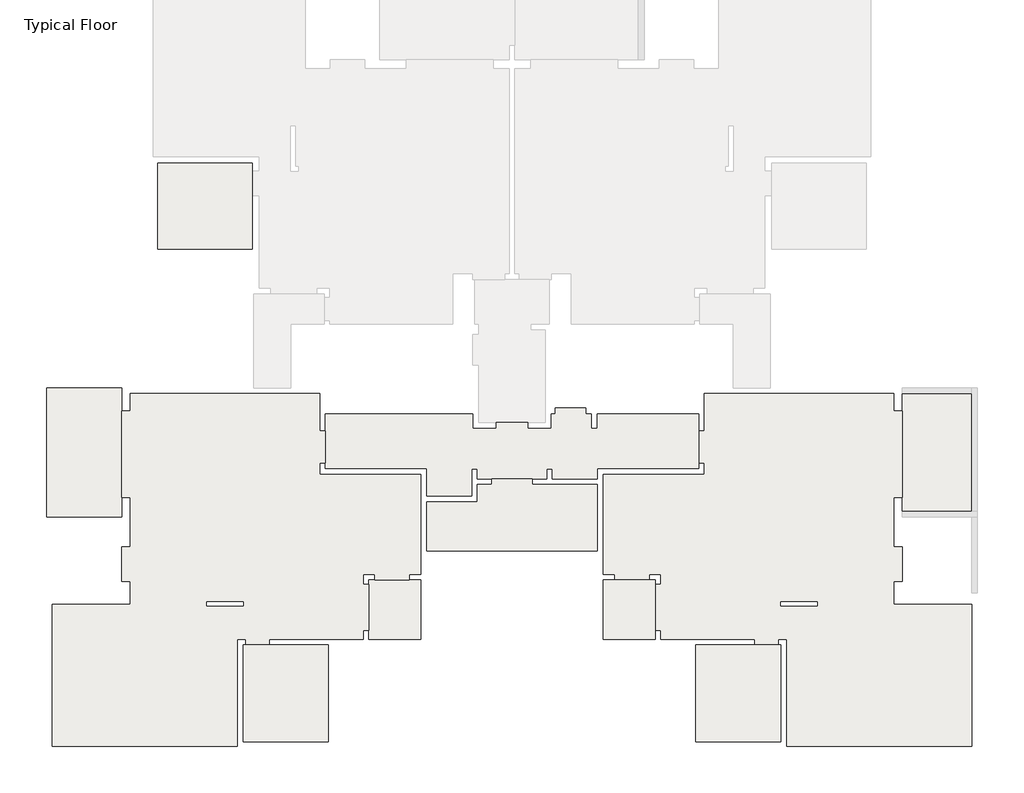
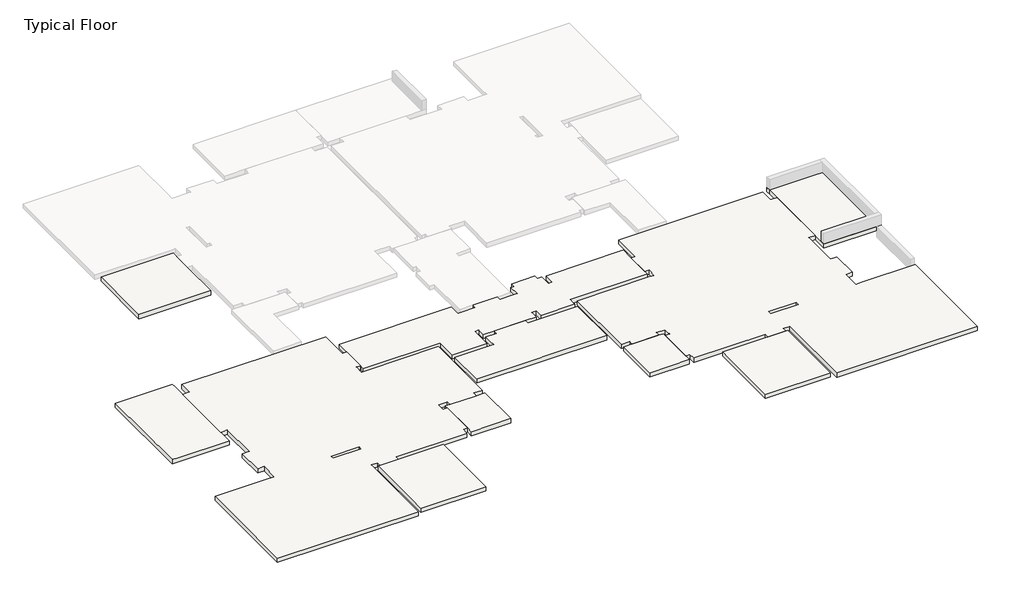
# One storey, part 1 of 2: 11 slabs.
"""IFC4 building model written with IfcOpenShell, lengths in millimetres."""

from ifc_helpers import new_model, si_unit, origin, place, context, project, spatial, faceted_brep, element, save

model = new_model("IFC4")

# Units and contexts
model_context = context("Model", 3, world=origin())
ifc_project = project(units=[si_unit("LENGTHUNIT", "METRE", prefix="MILLI")], contexts=[model_context])

# Site, building, storey
site = spatial("IfcSite", under=ifc_project)
building = spatial("IfcBuilding", under=site)
storey = spatial("IfcBuildingStorey", under=building, Name="Typical Floor", Elevation=3180.0)

# Slabs
placement = place(None, origin())
element("IfcSlab", 1, ObjectType="20", at=placement, inside=storey, context=model_context, shape_type="Brep", body=[
    faceted_brep([(-12093.8891281, 5078.7725736, 2980.0), (-12093.8891281, 8055.2636366, 2980.0), (-8823.7009813, 8055.2636366, 2980.0), (-8823.7009813, 7785.2636366, 2980.0), (-8823.7009813, 6932.7236554, 2980.0), (-8823.7009813, 5078.7725736, 2980.0), (-12093.8891281, 8055.2636366, 3180.0), (-12093.8891281, 5078.7725736, 3180.0), (-8823.7009813, 5078.7725736, 3180.0), (-8823.7009813, 6932.7236554, 3180.0), (-8823.7009813, 7785.2636366, 3180.0), (-8823.7009813, 8055.2636366, 3180.0)], [[[0, 1, 2, 3, 4, 5]], [[6, 7, 8, 9, 10, 11]], [[7, 0, 5, 8]], [[1, 0, 7, 6]], [[1, 6, 11, 2]], [[2, 11, 10, 9, 8, 5, 4, 3]]]),
])
element("IfcSlab", 2, ObjectType="20", at=placement, inside=storey, context=model_context, shape_type="Brep", body=[
    faceted_brep([(-15742.7132109, -12122.4503803, 2980.0), (-15742.7132109, -7221.2744631, 2980.0), (-13342.9013576, -7221.2744631, 2980.0), (-13042.9013576, -7221.2744631, 2980.0), (-13042.9013576, -6421.2274264, 2980.0), (-13342.9013576, -6421.2274264, 2980.0), (-13342.9013576, -5221.0863163, 2980.0), (-13042.9013576, -5221.0863163, 2980.0), (-13042.9013576, -3521.4155732, 2980.0), (-13342.9013576, -3521.4155732, 2980.0), (-13342.9013576, -517.8878215, 2980.0), (-13042.9013576, -517.8878215, 2980.0), (-13042.9013576, 79.007757, 2980.0), (-6495.0180086, 79.007757, 2980.0), (-6495.0180086, -1222.7326004, 2980.0), (-6295.0180086, -1222.7326004, 2980.0), (-6295.0180086, -2321.2744631, 2980.0), (-6493.9832015, -2321.2744631, 2980.0), (-6493.9832015, -2721.3214998, 2980.0), (-6293.9832015, -2721.3214998, 2980.0), (-2993.9832015, -2721.3214998, 2980.0), (-2993.9832015, -6171.4626098, 2980.0), (-3395.2061554, -6171.4626098, 2980.0), (-3395.2061554, -6371.4626098, 2980.0), (-4595.3472654, -6371.4626098, 2980.0), (-4595.3472654, -6171.4626098, 2980.0), (-4993.2776511, -6171.4626098, 2980.0), (-4993.2776511, -6371.4626098, 2980.0), (-4993.2776511, -6522.8266738, 2980.0), (-4793.2776511, -6522.8266738, 2980.0), (-4793.2776511, -8120.8981696, 2980.0), (-4993.2776511, -8120.8981696, 2980.0), (-4993.2776511, -8422.5444537, 2980.0), (-8238.1036154, -8422.5444537, 2980.0), (-8238.1036154, -8622.5444537, 2980.0), (-9048.7809437, -8622.5444537, 2980.0), (-9048.7809437, -8422.5444537, 2980.0), (-9343.7809437, -8422.5444537, 2980.0), (-9343.7809437, -8622.5444537, 2980.0), (-9343.7809437, -12122.4503803, 2980.0), (-9144.0302381, -7122.1211235, 2980.0), (-10394.9709719, -7122.1211235, 2980.0), (-10394.9709719, -7272.1211235, 2980.0), (-9144.0302381, -7272.1211235, 2980.0), (-15742.7132109, -7221.2744631, 3180.0), (-15742.7132109, -12122.4503803, 3180.0), (-9343.7809437, -12122.4503803, 3180.0), (-9343.7809437, -8622.5444537, 3180.0), (-9343.7809437, -8422.5444537, 3180.0), (-9048.7809437, -8422.5444537, 3180.0), (-9048.7809437, -8622.5444537, 3180.0), (-8238.1036154, -8622.5444537, 3180.0), (-8238.1036154, -8422.5444537, 3180.0), (-4993.2776511, -8422.5444537, 3180.0), (-4993.2776511, -8120.8981696, 3180.0), (-4793.2776511, -8120.8981696, 3180.0), (-4793.2776511, -6522.8266738, 3180.0), (-4993.2776511, -6522.8266738, 3180.0), (-4993.2776511, -6371.4626098, 3180.0), (-4993.2776511, -6171.4626098, 3180.0), (-4595.3472654, -6171.4626098, 3180.0), (-4595.3472654, -6371.4626098, 3180.0), (-3395.2061554, -6371.4626098, 3180.0), (-3395.2061554, -6171.4626098, 3180.0), (-2993.9832015, -6171.4626098, 3180.0), (-2993.9832015, -2721.3214998, 3180.0), (-6293.9832015, -2721.3214998, 3180.0), (-6493.9832015, -2721.3214998, 3180.0), (-6493.9832015, -2321.2744631, 3180.0), (-6295.0180086, -2321.2744631, 3180.0), (-6295.0180086, -1222.7326004, 3180.0), (-6495.0180086, -1222.7326004, 3180.0), (-6495.0180086, 79.007757, 3180.0), (-13042.9013576, 79.007757, 3180.0), (-13042.9013576, -517.8878215, 3180.0), (-13342.9013576, -517.8878215, 3180.0), (-13342.9013576, -3521.4155732, 3180.0), (-13042.9013576, -3521.4155732, 3180.0), (-13042.9013576, -5221.0863163, 3180.0), (-13342.9013576, -5221.0863163, 3180.0), (-13342.9013576, -6421.2274264, 3180.0), (-13042.9013576, -6421.2274264, 3180.0), (-13042.9013576, -7221.2744631, 3180.0), (-13342.9013576, -7221.2744631, 3180.0), (-10394.9709719, -7122.1211235, 3180.0), (-9144.0302381, -7122.1211235, 3180.0), (-9144.0302381, -7272.1211235, 3180.0), (-10394.9709719, -7272.1211235, 3180.0)], [[[0, 1, 2, 3, 4, 5, 6, 7, 8, 9, 10, 11, 12, 13, 14, 15, 16, 17, 18, 19, 20, 21, 22, 23, 24, 25, 26, 27, 28, 29, 30, 31, 32, 33, 34, 35, 36, 37, 38, 39], [40, 41, 42, 43]], [[44, 45, 46, 47, 48, 49, 50, 51, 52, 53, 54, 55, 56, 57, 58, 59, 60, 61, 62, 63, 64, 65, 66, 67, 68, 69, 70, 71, 72, 73, 74, 75, 76, 77, 78, 79, 80, 81, 82, 83], [84, 85, 86, 87]], [[1, 0, 45, 44]], [[1, 44, 83, 82, 3, 2]], [[4, 3, 82, 81]], [[5, 4, 81, 80]], [[6, 5, 80, 79]], [[7, 6, 79, 78]], [[8, 7, 78, 77]], [[9, 8, 77, 76]], [[10, 9, 76, 75]], [[11, 10, 75, 74]], [[12, 11, 74, 73]], [[13, 12, 73, 72]], [[14, 13, 72, 71]], [[15, 14, 71, 70]], [[16, 15, 70, 69]], [[17, 16, 69, 68]], [[18, 17, 68, 67]], [[18, 67, 66, 65, 20, 19]], [[21, 20, 65, 64]], [[22, 21, 64, 63]], [[23, 22, 63, 62]], [[24, 23, 62, 61]], [[25, 24, 61, 60]], [[26, 25, 60, 59]], [[26, 59, 58, 57, 28, 27]], [[29, 28, 57, 56]], [[30, 29, 56, 55]], [[31, 30, 55, 54]], [[32, 31, 54, 53]], [[33, 32, 53, 52]], [[34, 33, 52, 51]], [[35, 34, 51, 50]], [[36, 35, 50, 49]], [[37, 36, 49, 48]], [[37, 48, 47, 46, 39, 38]], [[0, 39, 46, 45]], [[41, 40, 85, 84]], [[42, 41, 84, 87]], [[43, 42, 87, 86]], [[40, 43, 86, 85]]]),
])
element("IfcSlab", 3, ObjectType="20", at=placement, inside=storey, context=model_context, shape_type="Brep", body=[
    faceted_brep([(-6193.7809437, -8622.5444537, 2980.0), (-6193.7809437, -11972.4503803, 2980.0), (-9143.7809437, -11972.4503803, 2980.0), (-9143.7809437, -8622.5444537, 2980.0), (-9048.7809437, -8622.5444537, 2980.0), (-8238.1036154, -8622.5444537, 2980.0), (-6193.7809437, -11972.4503803, 3180.0), (-6193.7809437, -8622.5444537, 3180.0), (-8238.1036154, -8622.5444537, 3180.0), (-9048.7809437, -8622.5444537, 3180.0), (-9143.7809437, -8622.5444537, 3180.0), (-9143.7809437, -11972.4503803, 3180.0)], [[[0, 1, 2, 3, 4, 5]], [[6, 7, 8, 9, 10, 11]], [[1, 0, 7, 6]], [[2, 1, 6, 11]], [[3, 2, 11, 10]], [[3, 10, 9, 8, 7, 0, 5, 4]]]),
])
element("IfcSlab", 4, ObjectType="20", at=placement, inside=storey, context=model_context, shape_type="Brep", body=[
    faceted_brep([(-13342.9013576, -4192.3939363, 2980.0), (-15942.7132109, -4192.3939363, 2980.0), (-15942.7132109, 279.007757, 2980.0), (-13343.4657979, 279.007757, 2980.0), (-13343.4657979, 79.007757, 2980.0), (-13342.9013576, 79.007757, 2980.0), (-13342.9013576, -517.8878215, 2980.0), (-13342.9013576, -3521.4155732, 2980.0), (-15942.7132109, -4192.3939363, 3180.0), (-15742.7132109, -4192.3939363, 3180.0), (-13342.9013576, -4192.3939363, 3180.0), (-13342.9013576, -3992.3939363, 3180.0), (-13342.9013576, -3521.4155732, 3180.0), (-13342.9013576, -517.8878215, 3180.0), (-13342.9013576, 79.007757, 3180.0), (-13343.4657979, 79.007757, 3180.0), (-13343.4657979, 279.007757, 3180.0), (-15742.7132109, 279.007757, 3180.0), (-15942.7132109, 279.007757, 3180.0)], [[[0, 1, 2, 3, 4, 5, 6, 7]], [[8, 9, 10, 11, 12, 13, 14, 15, 16, 17, 18]], [[10, 0, 7, 6, 5, 14, 13, 12, 11]], [[1, 0, 10, 9, 8]], [[2, 1, 8, 18]], [[2, 18, 17, 16, 3]], [[4, 15, 14, 5]], [[15, 4, 3, 16]]]),
])
element("IfcSlab", 5, ObjectType="20", at=placement, inside=storey, context=model_context, shape_type="Brep", body=[
    faceted_brep([(16056.8164223, -7221.2744631, 2980.0), (16056.8164223, -12122.4503803, 2980.0), (9657.8841551, -12122.4503803, 2980.0), (9657.8841551, -8622.5444537, 2980.0), (9657.8841551, -8422.5444537, 2980.0), (9362.8841551, -8422.5444537, 2980.0), (9362.8841551, -8622.5444537, 2980.0), (8552.2068268, -8622.5444537, 2980.0), (8552.2068268, -8422.5444537, 2980.0), (5307.3808625, -8422.5444537, 2980.0), (5307.3808625, -8120.8981696, 2980.0), (5107.3808625, -8120.8981696, 2980.0), (5107.3808625, -6522.8266738, 2980.0), (5307.3808625, -6522.8266738, 2980.0), (5307.3808625, -6371.4626098, 2980.0), (5307.3808625, -6171.4626098, 2980.0), (4909.4504768, -6171.4626098, 2980.0), (4909.4504768, -6371.4626098, 2980.0), (3709.3093668, -6371.4626098, 2980.0), (3709.3093668, -6171.4626098, 2980.0), (3308.0864128, -6171.4626098, 2980.0), (3308.0864128, -2721.3214998, 2980.0), (6608.0864128, -2721.3214998, 2980.0), (6808.0864128, -2721.3214998, 2980.0), (6808.0864128, -2321.2744631, 2980.0), (6609.12122, -2321.2744631, 2980.0), (6609.12122, -1222.7326004, 2980.0), (6809.12122, -1222.7326004, 2980.0), (6809.12122, 79.007757, 2980.0), (13357.004569, 79.007757, 2980.0), (13357.004569, -517.8878215, 2980.0), (13657.004569, -517.8878215, 2980.0), (13657.004569, -3521.4155732, 2980.0), (13357.004569, -3521.4155732, 2980.0), (13357.004569, -5221.0863163, 2980.0), (13657.004569, -5221.0863163, 2980.0), (13657.004569, -6421.2274264, 2980.0), (13357.004569, -6421.2274264, 2980.0), (13357.004569, -7221.2744631, 2980.0), (13657.004569, -7221.2744631, 2980.0), (10709.0741833, -7122.1211235, 2980.0), (9458.1334495, -7122.1211235, 2980.0), (9458.1334495, -7272.1211235, 2980.0), (10709.0741833, -7272.1211235, 2980.0), (16056.8164223, -12122.4503803, 3180.0), (16056.8164223, -7221.2744631, 3180.0), (13657.004569, -7221.2744631, 3180.0), (13357.004569, -7221.2744631, 3180.0), (13357.004569, -6421.2274264, 3180.0), (13657.004569, -6421.2274264, 3180.0), (13657.004569, -5221.0863163, 3180.0), (13357.004569, -5221.0863163, 3180.0), (13357.004569, -3521.4155732, 3180.0), (13657.004569, -3521.4155732, 3180.0), (13657.004569, -517.8878215, 3180.0), (13357.004569, -517.8878215, 3180.0), (13357.004569, 79.007757, 3180.0), (6809.12122, 79.007757, 3180.0), (6809.12122, -1222.7326004, 3180.0), (6609.12122, -1222.7326004, 3180.0), (6609.12122, -2321.2744631, 3180.0), (6808.0864128, -2321.2744631, 3180.0), (6808.0864128, -2721.3214998, 3180.0), (6608.0864128, -2721.3214998, 3180.0), (3308.0864128, -2721.3214998, 3180.0), (3308.0864128, -6171.4626098, 3180.0), (3709.3093668, -6171.4626098, 3180.0), (3709.3093668, -6371.4626098, 3180.0), (4909.4504768, -6371.4626098, 3180.0), (4909.4504768, -6171.4626098, 3180.0), (5307.3808625, -6171.4626098, 3180.0), (5307.3808625, -6371.4626098, 3180.0), (5307.3808625, -6522.8266738, 3180.0), (5107.3808625, -6522.8266738, 3180.0), (5107.3808625, -8120.8981696, 3180.0), (5307.3808625, -8120.8981696, 3180.0), (5307.3808625, -8422.5444537, 3180.0), (8552.2068268, -8422.5444537, 3180.0), (8552.2068268, -8622.5444537, 3180.0), (9362.8841551, -8622.5444537, 3180.0), (9362.8841551, -8422.5444537, 3180.0), (9657.8841551, -8422.5444537, 3180.0), (9657.8841551, -8622.5444537, 3180.0), (9657.8841551, -12122.4503803, 3180.0), (9458.1334495, -7122.1211235, 3180.0), (10709.0741833, -7122.1211235, 3180.0), (10709.0741833, -7272.1211235, 3180.0), (9458.1334495, -7272.1211235, 3180.0)], [[[0, 1, 2, 3, 4, 5, 6, 7, 8, 9, 10, 11, 12, 13, 14, 15, 16, 17, 18, 19, 20, 21, 22, 23, 24, 25, 26, 27, 28, 29, 30, 31, 32, 33, 34, 35, 36, 37, 38, 39], [40, 41, 42, 43]], [[44, 45, 46, 47, 48, 49, 50, 51, 52, 53, 54, 55, 56, 57, 58, 59, 60, 61, 62, 63, 64, 65, 66, 67, 68, 69, 70, 71, 72, 73, 74, 75, 76, 77, 78, 79, 80, 81, 82, 83], [84, 85, 86, 87]], [[1, 0, 45, 44]], [[38, 47, 46, 45, 0, 39]], [[38, 37, 48, 47]], [[37, 36, 49, 48]], [[36, 35, 50, 49]], [[35, 34, 51, 50]], [[34, 33, 52, 51]], [[33, 32, 53, 52]], [[32, 31, 54, 53]], [[31, 30, 55, 54]], [[30, 29, 56, 55]], [[29, 28, 57, 56]], [[28, 27, 58, 57]], [[27, 26, 59, 58]], [[26, 25, 60, 59]], [[25, 24, 61, 60]], [[24, 23, 62, 61]], [[21, 64, 63, 62, 23, 22]], [[21, 20, 65, 64]], [[20, 19, 66, 65]], [[19, 18, 67, 66]], [[18, 17, 68, 67]], [[17, 16, 69, 68]], [[16, 15, 70, 69]], [[13, 72, 71, 70, 15, 14]], [[13, 12, 73, 72]], [[12, 11, 74, 73]], [[11, 10, 75, 74]], [[10, 9, 76, 75]], [[9, 8, 77, 76]], [[8, 7, 78, 77]], [[7, 6, 79, 78]], [[6, 5, 80, 79]], [[5, 4, 81, 80]], [[2, 83, 82, 81, 4, 3]], [[2, 1, 44, 83]], [[41, 40, 85, 84]], [[40, 43, 86, 85]], [[43, 42, 87, 86]], [[42, 41, 84, 87]]]),
])
element("IfcSlab", 6, ObjectType="20", at=placement, inside=storey, context=model_context, shape_type="Brep", body=[
    faceted_brep([(6507.8841551, -11972.4503803, 2980.0), (6507.8841551, -8622.5444537, 2980.0), (8552.2068268, -8622.5444537, 2980.0), (9362.8841551, -8622.5444537, 2980.0), (9457.8841551, -8622.5444537, 2980.0), (9457.8841551, -11972.4503803, 2980.0), (6507.8841551, -8622.5444537, 3180.0), (6507.8841551, -11972.4503803, 3180.0), (9457.8841551, -11972.4503803, 3180.0), (9457.8841551, -8622.5444537, 3180.0), (9362.8841551, -8622.5444537, 3180.0), (8552.2068268, -8622.5444537, 3180.0)], [[[0, 1, 2, 3, 4, 5]], [[6, 7, 8, 9, 10, 11]], [[1, 0, 7, 6]], [[0, 5, 8, 7]], [[5, 4, 9, 8]], [[9, 4, 3, 2, 1, 6, 11, 10]]]),
])
element("IfcSlab", 7, ObjectType="20", at=placement, inside=storey, context=model_context, shape_type="Brep", body=[
    faceted_brep([(16256.8164223, -4192.3939363, 2980.0), (13657.004569, -4192.3939363, 2980.0), (13657.004569, -3521.4155732, 2980.0), (13657.004569, -517.8878215, 2980.0), (13657.004569, 79.007757, 2980.0), (13657.5690093, 79.007757, 2980.0), (13657.5690093, 279.007757, 2980.0), (16256.8164223, 279.007757, 2980.0), (13657.004569, -4192.3939363, 3180.0), (16056.8164223, -4192.3939363, 3180.0), (16256.8164223, -4192.3939363, 3180.0), (16256.8164223, -3992.3939363, 3180.0), (16256.8164223, 279.007757, 3180.0), (16056.8164223, 279.007757, 3180.0), (13657.5690093, 279.007757, 3180.0), (13657.5690093, 79.007757, 3180.0), (13657.004569, 79.007757, 3180.0), (13657.004569, -517.8878215, 3180.0), (13657.004569, -3521.4155732, 3180.0), (13657.004569, -3992.3939363, 3180.0)], [[[0, 1, 2, 3, 4, 5, 6, 7]], [[8, 9, 10, 11, 12, 13, 14, 15, 16, 17, 18, 19]], [[1, 8, 19, 18, 17, 16, 4, 3, 2]], [[1, 0, 10, 9, 8]], [[0, 7, 12, 11, 10]], [[12, 7, 6, 14, 13]], [[15, 5, 4, 16]], [[5, 15, 14, 6]]]),
])
element("IfcSlab", 8, ObjectType="20", at=placement, inside=storey, context=model_context, shape_type="Brep", body=[
    faceted_brep([(-2793.9832015, -3671.6977933, 2980.0), (-1043.6069079, -3671.6977933, 2980.0), (-1043.6069079, -3471.6977933, 2980.0), (-1043.6069079, -3071.6037199, 2980.0), (-544.0772748, -3071.6037199, 2980.0), (-544.0772748, -2871.6037199, 2980.0), (857.1456791, -2871.6037199, 2980.0), (857.1456791, -2872.6855637, 2980.0), (857.1456791, -3072.6855637, 2980.0), (3108.0864128, -3072.6855637, 2980.0), (3108.0864128, -5372.4503803, 2980.0), (-2793.9832015, -5372.4503803, 2980.0), (-1043.6069079, -3671.6977933, 3180.0), (-2793.9832015, -3671.6977933, 3180.0), (-2793.9832015, -5372.4503803, 3180.0), (3108.0864128, -5372.4503803, 3180.0), (3108.0864128, -3072.6855637, 3180.0), (857.1456791, -3072.6855637, 3180.0), (857.1456791, -2872.6855637, 3180.0), (857.1456791, -2871.6037199, 3180.0), (-544.0772748, -2871.6037199, 3180.0), (-544.0772748, -3071.6037199, 3180.0), (-1043.6069079, -3071.6037199, 3180.0), (-1043.6069079, -3471.6977933, 3180.0)], [[[0, 1, 2, 3, 4, 5, 6, 7, 8, 9, 10, 11]], [[12, 13, 14, 15, 16, 17, 18, 19, 20, 21, 22, 23]], [[1, 0, 13, 12]], [[1, 12, 23, 22, 3, 2]], [[4, 3, 22, 21]], [[5, 4, 21, 20]], [[6, 5, 20, 19]], [[6, 19, 18, 17, 8, 7]], [[9, 8, 17, 16]], [[10, 9, 16, 15]], [[11, 10, 15, 14]], [[0, 11, 14, 13]]]),
])
element("IfcSlab", 9, ObjectType="20", at=placement, inside=storey, context=model_context, shape_type="Brep", body=[
    faceted_brep([(-6295.0180086, -621.6037199, 2980.0), (-1194.9239352, -621.6037199, 2980.0), (-1194.9239352, -1121.133353, 2980.0), (-994.9239352, -1121.133353, 2980.0), (-393.7950547, -1121.133353, 2980.0), (-393.7950547, -921.133353, 2980.0), (707.8982661, -921.133353, 2980.0), (707.8982661, -1121.133353, 2980.0), (1309.0271466, -1121.133353, 2980.0), (1509.0271466, -1121.133353, 2980.0), (1509.0271466, -622.6385271, 2980.0), (1655.1231015, -622.6385271, 2980.0), (1655.1231015, -422.6385271, 2980.0), (1655.1231015, -421.6037199, 2980.0), (2709.12122, -421.6037199, 2980.0), (2709.12122, -621.6037199, 2980.0), (2906.0638352, -621.6037199, 2980.0), (2906.0638352, -1121.133353, 2980.0), (3106.0638352, -1121.133353, 2980.0), (3106.0638352, -621.6037199, 2980.0), (6609.12122, -621.6037199, 2980.0), (6609.12122, -1222.7326004, 2980.0), (6609.12122, -2321.2744631, 2980.0), (6608.0864128, -2321.2744631, 2980.0), (6608.0864128, -2521.3214998, 2980.0), (3108.0864128, -2521.3214998, 2980.0), (3108.0864128, -2721.3214998, 2980.0), (3108.0864128, -2872.6855637, 2980.0), (1555.640505, -2872.6855637, 2980.0), (1555.640505, -2522.3563069, 2980.0), (1355.640505, -2522.3563069, 2980.0), (1355.640505, -2872.6855637, 2980.0), (857.1456791, -2872.6855637, 2980.0), (857.1456791, -2871.6037199, 2980.0), (-544.0772748, -2871.6037199, 2980.0), (-1043.6069079, -2871.6037199, 2980.0), (-1043.6069079, -2526.6037199, 2980.0), (-1243.6069079, -2526.6037199, 2980.0), (-1243.6069079, -3471.6977933, 2980.0), (-2793.9832015, -3471.6977933, 2980.0), (-2793.9832015, -2721.3214998, 2980.0), (-2793.9832015, -2521.3214998, 2980.0), (-6293.9832015, -2521.3214998, 2980.0), (-6293.9832015, -2321.2744631, 2980.0), (-6295.0180086, -2321.2744631, 2980.0), (-6295.0180086, -1222.7326004, 2980.0), (-1194.9239352, -621.6037199, 3180.0), (-6295.0180086, -621.6037199, 3180.0), (-6295.0180086, -1222.7326004, 3180.0), (-6295.0180086, -2321.2744631, 3180.0), (-6293.9832015, -2321.2744631, 3180.0), (-6293.9832015, -2521.3214998, 3180.0), (-2793.9832015, -2521.3214998, 3180.0), (-2793.9832015, -2721.3214998, 3180.0), (-2793.9832015, -3471.6977933, 3180.0), (-1243.6069079, -3471.6977933, 3180.0), (-1243.6069079, -2526.6037199, 3180.0), (-1043.6069079, -2526.6037199, 3180.0), (-1043.6069079, -2871.6037199, 3180.0), (-544.0772748, -2871.6037199, 3180.0), (857.1456791, -2871.6037199, 3180.0), (857.1456791, -2872.6855637, 3180.0), (1355.640505, -2872.6855637, 3180.0), (1355.640505, -2522.3563069, 3180.0), (1555.640505, -2522.3563069, 3180.0), (1555.640505, -2872.6855637, 3180.0), (3108.0864128, -2872.6855637, 3180.0), (3108.0864128, -2721.3214998, 3180.0), (3108.0864128, -2521.3214998, 3180.0), (6608.0864128, -2521.3214998, 3180.0), (6608.0864128, -2321.2744631, 3180.0), (6609.12122, -2321.2744631, 3180.0), (6609.12122, -1222.7326004, 3180.0), (6609.12122, -621.6037199, 3180.0), (3106.0638352, -621.6037199, 3180.0), (3106.0638352, -1121.133353, 3180.0), (2906.0638352, -1121.133353, 3180.0), (2906.0638352, -621.6037199, 3180.0), (2709.12122, -621.6037199, 3180.0), (2709.12122, -421.6037199, 3180.0), (1655.1231015, -421.6037199, 3180.0), (1655.1231015, -422.6385271, 3180.0), (1655.1231015, -622.6385271, 3180.0), (1509.0271466, -622.6385271, 3180.0), (1509.0271466, -1121.133353, 3180.0), (1309.0271466, -1121.133353, 3180.0), (707.8982661, -1121.133353, 3180.0), (707.8982661, -921.133353, 3180.0), (-393.7950547, -921.133353, 3180.0), (-393.7950547, -1121.133353, 3180.0), (-994.9239352, -1121.133353, 3180.0), (-1194.9239352, -1121.133353, 3180.0)], [[[0, 1, 2, 3, 4, 5, 6, 7, 8, 9, 10, 11, 12, 13, 14, 15, 16, 17, 18, 19, 20, 21, 22, 23, 24, 25, 26, 27, 28, 29, 30, 31, 32, 33, 34, 35, 36, 37, 38, 39, 40, 41, 42, 43, 44, 45]], [[46, 47, 48, 49, 50, 51, 52, 53, 54, 55, 56, 57, 58, 59, 60, 61, 62, 63, 64, 65, 66, 67, 68, 69, 70, 71, 72, 73, 74, 75, 76, 77, 78, 79, 80, 81, 82, 83, 84, 85, 86, 87, 88, 89, 90, 91]], [[47, 0, 45, 44, 49, 48]], [[1, 0, 47, 46]], [[2, 1, 46, 91]], [[2, 91, 90, 89, 4, 3]], [[5, 4, 89, 88]], [[6, 5, 88, 87]], [[7, 6, 87, 86]], [[7, 86, 85, 84, 9, 8]], [[10, 9, 84, 83]], [[11, 10, 83, 82]], [[11, 82, 81, 80, 13, 12]], [[14, 13, 80, 79]], [[15, 14, 79, 78]], [[16, 15, 78, 77]], [[17, 16, 77, 76]], [[18, 17, 76, 75]], [[19, 18, 75, 74]], [[20, 19, 74, 73]], [[20, 73, 72, 71, 22, 21]], [[68, 25, 24, 69]], [[25, 68, 67, 66, 27, 26]], [[28, 27, 66, 65]], [[29, 28, 65, 64]], [[30, 29, 64, 63]], [[31, 30, 63, 62]], [[31, 62, 61, 32]], [[57, 36, 35, 58]], [[37, 36, 57, 56]], [[38, 37, 56, 55]], [[39, 38, 55, 54]], [[39, 54, 53, 52, 41, 40]], [[41, 52, 51, 42]], [[33, 60, 59, 58, 35, 34]], [[60, 33, 32, 61]], [[50, 43, 42, 51]], [[43, 50, 49, 44]], [[23, 70, 69, 24]], [[70, 23, 22, 71]]]),
])
element("IfcSlab", 10, ObjectType="20", at=placement, inside=storey, context=model_context, shape_type="Brep", body=[
    faceted_brep([(-2993.9832015, -6371.4626098, 2980.0), (-2993.9832015, -8420.9452063, 2980.0), (-4793.2776511, -8420.9452063, 2980.0), (-4793.2776511, -8120.8981696, 2980.0), (-4793.2776511, -6522.8266738, 2980.0), (-4793.2776511, -6371.4626098, 2980.0), (-4595.3472654, -6371.4626098, 2980.0), (-3395.2061554, -6371.4626098, 2980.0), (-2993.9832015, -8420.9452063, 3180.0), (-2993.9832015, -6371.4626098, 3180.0), (-3395.2061554, -6371.4626098, 3180.0), (-4595.3472654, -6371.4626098, 3180.0), (-4793.2776511, -6371.4626098, 3180.0), (-4793.2776511, -6522.8266738, 3180.0), (-4793.2776511, -8120.8981696, 3180.0), (-4793.2776511, -8420.9452063, 3180.0)], [[[0, 1, 2, 3, 4, 5, 6, 7]], [[8, 9, 10, 11, 12, 13, 14, 15]], [[1, 0, 9, 8]], [[2, 1, 8, 15]], [[2, 15, 14, 13, 12, 5, 4, 3]], [[5, 12, 11, 10, 9, 0, 7, 6]]]),
])
element("IfcSlab", 11, ObjectType="20", at=placement, inside=storey, context=model_context, shape_type="Brep", body=[
    faceted_brep([(3308.0864128, -8420.9495778, 2980.0), (3308.0864128, -6371.4626098, 2980.0), (3709.3093668, -6371.4626098, 2980.0), (4909.4504768, -6371.4626098, 2980.0), (5107.3808625, -6371.4626098, 2980.0), (5107.3808625, -6522.8266738, 2980.0), (5107.3808625, -8120.8981696, 2980.0), (5107.3808625, -8420.9495778, 2980.0), (3308.0864128, -6371.4626098, 3180.0), (3308.0864128, -8420.9495778, 3180.0), (5107.3808625, -8420.9495778, 3180.0), (5107.3808625, -8120.8981696, 3180.0), (5107.3808625, -6522.8266738, 3180.0), (5107.3808625, -6371.4626098, 3180.0), (4909.4504768, -6371.4626098, 3180.0), (3709.3093668, -6371.4626098, 3180.0)], [[[0, 1, 2, 3, 4, 5, 6, 7]], [[8, 9, 10, 11, 12, 13, 14, 15]], [[1, 0, 9, 8]], [[4, 13, 12, 11, 10, 7, 6, 5]], [[13, 4, 3, 2, 1, 8, 15, 14]], [[0, 7, 10, 9]]]),
])

save(model, "model.ifc")

# Revit data of these elements
# Type "20"
#   Type IfcGUID = "1zn3TUKgbD69x5FAYjkTF1"
#   Function = 0
#   Layers, outside or top first: 20 cm "Concrete" (function 1)
# Element 1 (IfcSlab, "20")
#   IfcGUID = "1e7LVzuKbECxrDX1g1kJq7"
#   Mark = "S2"
#   SOFiSTiK_AMG_Comments = ""
#   Height Offset From Level = 0 cm
#   built-in parameter 1001954 = 1
#   SOFiSTiK_AMG_Scheduled = yes
#   SOFiSTiK_AMG_Adjusted = yes
#   Phase Created = New Construction
#   Materials on its faces: "Concrete"
# Element 2 (IfcSlab, "20")
#   IfcGUID = "1e7LVzuKbECxrDX1g1kJrI"
#   Mark = "S3"
#   SOFiSTiK_AMG_Comments = ""
#   built-in parameter 1001955 = 3.14159 (stored number, unit not read)
#   Height Offset From Level = 0 cm
#   built-in parameter 1001954 = 1
#   SOFiSTiK_AMG_Scheduled = yes
#   SOFiSTiK_AMG_Adjusted = yes
#   Phase Created = New Construction
#   Materials on its faces: "Concrete"
# Element 3 (IfcSlab, "20")
#   IfcGUID = "3brXM_Qu1DvOaG$o2DBDiT"
#   Mark = "S4"
#   SOFiSTiK_AMG_Comments = ""
#   Height Offset From Level = 0 cm
#   built-in parameter 1001954 = 1
#   SOFiSTiK_AMG_Scheduled = yes
#   SOFiSTiK_AMG_Adjusted = yes
#   Phase Created = New Construction
#   Materials on its faces: "Concrete"
# Element 4 (IfcSlab, "20")
#   IfcGUID = "3brXM_Qu1DvOaG$o2DBDMY"
#   Mark = "S5"
#   SOFiSTiK_AMG_Comments = ""
#   Height Offset From Level = 0 cm
#   built-in parameter 1001954 = 1
#   SOFiSTiK_AMG_Scheduled = yes
#   SOFiSTiK_AMG_Adjusted = yes
#   Phase Created = New Construction
#   Materials on its faces: "Concrete"
# Element 5 (IfcSlab, "20")
#   IfcGUID = "3brXM_Qu1DvOaG$o2DBD3Y"
#   Mark = "S9"
#   SOFiSTiK_AMG_Comments = ""
#   built-in parameter 1001955 = 0 (stored number, unit not read)
#   Height Offset From Level = 0 cm
#   built-in parameter 1001954 = 1
#   SOFiSTiK_AMG_Scheduled = yes
#   SOFiSTiK_AMG_Adjusted = yes
#   Phase Created = New Construction
#   Materials on its faces: "Concrete"
# Element 6 (IfcSlab, "20")
#   IfcGUID = "3brXM_Qu1DvOaG$o2DBD4h"
#   Mark = "S10"
#   SOFiSTiK_AMG_Comments = ""
#   built-in parameter 1001955 = 3.14159 (stored number, unit not read)
#   Height Offset From Level = 0 cm
#   built-in parameter 1001954 = 1
#   SOFiSTiK_AMG_Scheduled = yes
#   SOFiSTiK_AMG_Adjusted = yes
#   Phase Created = New Construction
#   Materials on its faces: "Concrete"
# Element 7 (IfcSlab, "20")
#   IfcGUID = "3brXM_Qu1DvOaG$o2DBD48"
#   Mark = "S11"
#   SOFiSTiK_AMG_Comments = ""
#   built-in parameter 1001955 = 3.14159 (stored number, unit not read)
#   Height Offset From Level = 0 cm
#   built-in parameter 1001954 = 1
#   SOFiSTiK_AMG_Scheduled = yes
#   SOFiSTiK_AMG_Adjusted = yes
#   Phase Created = New Construction
#   Materials on its faces: "Concrete"
# Element 8 (IfcSlab, "20")
#   IfcGUID = "3brXM_Qu1DvOaG$o2DB2kd"
#   Mark = "S12"
#   SOFiSTiK_AMG_Comments = ""
#   built-in parameter 1001955 = 1.5708 (stored number, unit not read)
#   Height Offset From Level = 0 cm
#   built-in parameter 1001954 = 1
#   SOFiSTiK_AMG_Scheduled = yes
#   SOFiSTiK_AMG_Adjusted = yes
#   Phase Created = New Construction
#   Materials on its faces: "Concrete"
# Element 9 (IfcSlab, "20")
#   IfcGUID = "3brXM_Qu1DvOaG$o2DB2NX"
#   Mark = "S13"
#   SOFiSTiK_AMG_Comments = ""
#   built-in parameter 1001955 = -1.5708 (stored number, unit not read)
#   Height Offset From Level = 0 cm
#   built-in parameter 1001954 = 1
#   SOFiSTiK_AMG_Scheduled = yes
#   SOFiSTiK_AMG_Adjusted = yes
#   Phase Created = New Construction
#   Materials on its faces: "Concrete"
# Element 10 (IfcSlab, "20")
#   IfcGUID = "3brXM_Qu1DvOaG$o2DB3Nw"
#   Mark = "S17"
#   SOFiSTiK_AMG_Comments = ""
#   Height Offset From Level = 0 cm
#   built-in parameter 1001954 = 1
#   SOFiSTiK_AMG_Scheduled = yes
#   SOFiSTiK_AMG_Adjusted = yes
#   Phase Created = New Construction
#   Materials on its faces: "Concrete"
# Element 11 (IfcSlab, "20")
#   IfcGUID = "3brXM_Qu1DvOaG$o2DB3N9"
#   Mark = "S18"
#   SOFiSTiK_AMG_Comments = ""
#   built-in parameter 1001955 = 3.14159 (stored number, unit not read)
#   Height Offset From Level = 0 cm
#   built-in parameter 1001954 = 1
#   SOFiSTiK_AMG_Scheduled = yes
#   SOFiSTiK_AMG_Adjusted = yes
#   Phase Created = New Construction
#   Materials on its faces: "Concrete"
# Materials
#   "Concrete": class "Concrete", colour RGB 192 192 192, transparency 0, Keynote = "01000", Description = "Cast-in-place concrete", Cost = 0
